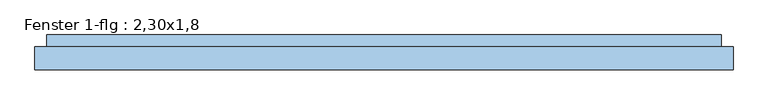
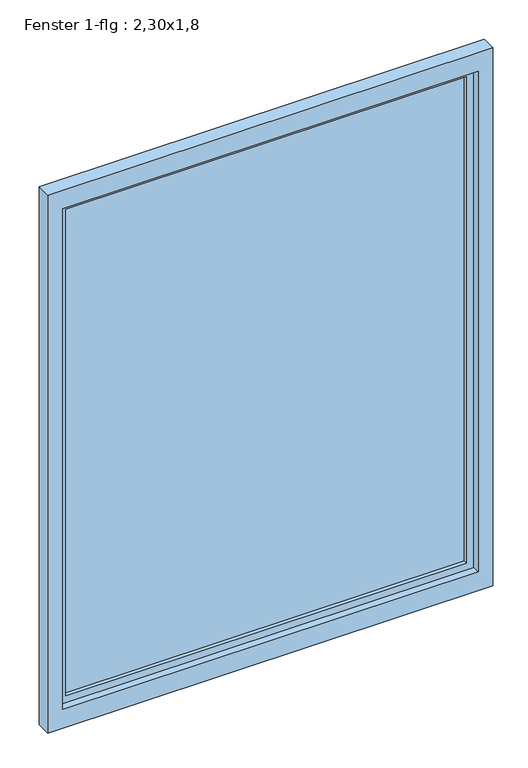
"""IFC4 building model written with IfcOpenShell, lengths in millimetres: window geometry, Fenster 1-flg : 2,30x1,8."""

import ifcopenshell
import ifcopenshell.guid

model = None  # the IFC model being written
_history = None  # IfcOwnerHistory: only IFC2X3 demands one
_inside = {}  # id of a spatial element -> (the spatial element, [elements in it])
_under = {}  # id of a project, library or spatial element -> (it, [spatial elements below it])
_declared = {}  # id of a project -> (the project, [libraries it declares])
_typed = {}  # id of a type object -> (the type object, [elements of that type])
_made_of = {}  # id of a material, layer set ... -> (it, [elements and type objects made of it])


def new_model(schema):
    """Start an empty IFC model of exactly this schema.

    Asked for "IFC4X3", IfcOpenShell would pick the latest addendum, in which some entities
    have other attributes; the version numbers below select the first issue.
    IFC2X3 requires an IfcOwnerHistory on every rooted entity: one is made here for all.
    """
    global model, _history
    if schema == "IFC4X3":
        model = ifcopenshell.file(schema_version=(4, 3, 0, 0))
    else:
        model = ifcopenshell.file(schema=schema)
    _inside.clear()
    _under.clear()
    _declared.clear()
    _typed.clear()
    _made_of.clear()
    _history = None
    if model.schema == "IFC2X3":
        org = make("IfcOrganization", Name="unknown")
        user = make(
            "IfcPersonAndOrganization",
            ThePerson=make("IfcPerson", FamilyName="unknown"),
            TheOrganization=org,
        )
        app = make(
            "IfcApplication",
            ApplicationDeveloper=org,
            Version="unknown",
            ApplicationFullName="unknown",
            ApplicationIdentifier="unknown",
        )
        _history = make(
            "IfcOwnerHistory",
            OwningUser=user,
            OwningApplication=app,
            ChangeAction="ADDED",
            CreationDate=0,
        )
    return model


def make(cls, **values):
    """One entity of the class cls with the attributes given. An attribute that is None is left unset."""
    return model.create_entity(
        cls, **{name: value for name, value in values.items() if value is not None}
    )


def rooted(cls, **values):
    """An entity with a GlobalId (a new one), such as an element, a storey or a relation."""
    return make(cls, GlobalId=ifcopenshell.guid.new(), OwnerHistory=_history, **values)


def si_unit(unit_type, name, prefix=None):
    """IfcSIUnit, for example si_unit("LENGTHUNIT", "METRE", prefix="MILLI")."""
    return make("IfcSIUnit", UnitType=unit_type, Prefix=prefix, Name=name)


def assignment(units):
    """IfcUnitAssignment: the units of a project."""
    return None if units is None else make("IfcUnitAssignment", Units=units)


def point(xyz):
    """IfcCartesianPoint."""
    return None if xyz is None else make("IfcCartesianPoint", Coordinates=xyz)


def direction(xyz):
    """IfcDirection."""
    return None if xyz is None else make("IfcDirection", DirectionRatios=xyz)


def frame(location, z_axis=None, x_axis=None):
    """IfcAxis2Placement3D, a coordinate frame: its origin and axes. An axis left out is left unset."""
    return make(
        "IfcAxis2Placement3D",
        Location=point(location),
        Axis=direction(z_axis),
        RefDirection=direction(x_axis),
    )


def origin():
    """The frame at (0, 0, 0) with its axes left unset."""
    return frame((0.0, 0.0, 0.0))


def place(relative_to, where):
    """IfcLocalPlacement: puts the frame where relative to a parent placement (None: the world)."""
    return make(
        "IfcLocalPlacement", PlacementRelTo=relative_to, RelativePlacement=where
    )


def context(
    kind, dimensions, precision=None, world=None, true_north=None, identifier=None
):
    """IfcGeometricRepresentationContext, for example the 3D "Model" context."""
    return make(
        "IfcGeometricRepresentationContext",
        ContextIdentifier=identifier,
        ContextType=kind,
        CoordinateSpaceDimension=dimensions,
        Precision=precision,
        WorldCoordinateSystem=world,
        TrueNorth=true_north,
    )


def project(units=None, contexts=None):
    """IfcProject with its units and contexts."""
    return rooted(
        "IfcProject",
        Name="project",
        RepresentationContexts=contexts,
        UnitsInContext=assignment(units),
    )


def spatial(cls, under=None, at=None, **own):
    """A site, building, storey or space (cls), placed at a placement, below another one or the project."""
    s = rooted(cls, ObjectPlacement=at, **own)
    if under is not None:
        _under.setdefault(under.id(), (under, []))[1].append(s)
    return s


def polyline(points):
    """IfcPolyline through the points."""
    return make("IfcPolyline", Points=[point(p) for p in points])


def outline(outer, holes=None, kind="AREA"):
    """IfcArbitraryClosedProfileDef: a profile drawn as a closed curve; with holes, ...WithVoids."""
    if holes is None:
        return make("IfcArbitraryClosedProfileDef", ProfileType=kind, OuterCurve=outer)
    return make(
        "IfcArbitraryProfileDefWithVoids",
        ProfileType=kind,
        OuterCurve=outer,
        InnerCurves=holes,
    )


def extrude(swept, where, along, depth):
    """IfcExtrudedAreaSolid: the profile swept, set in the frame where, extruded along a direction by depth."""
    return make(
        "IfcExtrudedAreaSolid",
        SweptArea=swept,
        Position=where,
        ExtrudedDirection=direction(along),
        Depth=depth,
    )


def faces_of(points, faces, orient=None, outer=None):
    """IfcFace entities. A face is a list of loops; a loop is a list of indices into points, from 0.

    orient and outer hold one flag for each loop. By default every Orientation is true, the
    first loop of a face is its IfcFaceOuterBound and the others are IfcFaceBound.
    """
    made = []
    for i, loops in enumerate(faces):
        bounds = []
        for j, loop in enumerate(loops):
            is_outer = j == 0 if outer is None else outer[i][j]
            bounds.append(
                make(
                    "IfcFaceOuterBound" if is_outer else "IfcFaceBound",
                    Bound=make("IfcPolyLoop", Polygon=[points[k] for k in loop]),
                    Orientation=True if orient is None else orient[i][j],
                )
            )
        made.append(make("IfcFace", Bounds=bounds))
    return made


def faceted_brep(points, faces, orient=None, outer=None, voids=None):
    """IfcFacetedBrep: a solid bounded by flat faces; with voids (closed shells), ...WithVoids."""
    shared = [point(p) for p in points]
    hull = make("IfcClosedShell", CfsFaces=faces_of(shared, faces, orient, outer))
    if voids is None:
        return make("IfcFacetedBrep", Outer=hull)
    return make(
        "IfcFacetedBrepWithVoids",
        Outer=hull,
        Voids=[
            make(cls, CfsFaces=faces_of(shared, fs, o, b)) for cls, fs, o, b in voids
        ],
    )


def shape(context_of_items, identifier, shape_type, items):
    """IfcShapeRepresentation: the items that make up one representation, for example the "Body"."""
    return make(
        "IfcShapeRepresentation",
        ContextOfItems=context_of_items,
        RepresentationIdentifier=identifier,
        RepresentationType=shape_type,
        Items=items,
    )


def source(mapping_origin, context_of_items, identifier, shape_type, items):
    """IfcRepresentationMap: a shape defined once, which mapped items show again and again."""
    return make(
        "IfcRepresentationMap",
        MappingOrigin=mapping_origin,
        MappedRepresentation=shape(context_of_items, identifier, shape_type, items),
    )


def transform(
    local_origin,
    x_axis=None,
    y_axis=None,
    z_axis=None,
    scale=None,
    scale2=None,
    scale3=None,
    uniform=True,
):
    """IfcCartesianTransformationOperator3D, or its non-uniform kind. x_axis, y_axis, z_axis: its Axis1, 2, 3."""
    if uniform:
        return make(
            "IfcCartesianTransformationOperator3D",
            Axis1=direction(x_axis),
            Axis2=direction(y_axis),
            LocalOrigin=point(local_origin),
            Scale=scale,
            Axis3=direction(z_axis),
        )
    return make(
        "IfcCartesianTransformationOperator3DnonUniform",
        Axis1=direction(x_axis),
        Axis2=direction(y_axis),
        LocalOrigin=point(local_origin),
        Scale=scale,
        Axis3=direction(z_axis),
        Scale2=scale2,
        Scale3=scale3,
    )


def mapped(mapping_source, mapping_target):
    """IfcMappedItem: shows the shape of a source again, moved by a transform."""
    return make(
        "IfcMappedItem", MappingSource=mapping_source, MappingTarget=mapping_target
    )


def made_of(thing, what):
    """Note that an element or type object is made of a material, layer set ...; save() writes the relation."""
    if what is not None:
        _made_of.setdefault(what.id(), (what, []))[1].append(thing)
    return thing


def element(
    cls,
    number,
    at=None,
    inside=None,
    cuts=None,
    type_object=None,
    material=None,
    context=None,
    identifier="Body",
    shape_type=None,
    held_by="IfcProductDefinitionShape",
    body=None,
    shapes=None,
    **own,
):
    """One element of the class cls, such as IfcWall. Its Tag is "e" and its number.

    at: its placement. inside: the storey or other place that contains it. cuts: it is an
    opening in that element (IfcRelVoidsElement). A single representation is given by context,
    identifier, shape_type and body (its items); several are given by shapes. held_by: the class
    of the entity that holds the representations. save() writes the other relations.
    """
    e = rooted(cls, Tag="e%d" % number, ObjectPlacement=at, **own)
    if body is not None:
        shapes = [shape(context, identifier, shape_type, body)]
    if shapes is not None:
        e.Representation = make(held_by, Representations=shapes)
    if inside is not None:
        _inside.setdefault(inside.id(), (inside, []))[1].append(e)
    if cuts is not None:
        rooted(
            "IfcRelVoidsElement", RelatingBuildingElement=cuts, RelatedOpeningElement=e
        )
    if type_object is not None:
        _typed.setdefault(type_object.id(), (type_object, []))[1].append(e)
    return made_of(e, material)


def aggregate(whole, parts):
    """IfcRelAggregates: a whole, such as a stair, and the parts it consists of."""
    return rooted("IfcRelAggregates", RelatingObject=whole, RelatedObjects=parts)


def save(model, path):
    """Write the relations noted so far, then the file.

    IfcRelAggregates (storeys below a building ...), IfcRelContainedInSpatialStructure (elements
    in a storey), IfcRelDefinesByType, IfcRelAssociatesMaterial and IfcRelDeclares: one each for
    every whole, place, type object, material and project.
    """
    for whole, parts in _under.values():
        aggregate(whole, parts)
    for where, things in _inside.values():
        rooted(
            "IfcRelContainedInSpatialStructure",
            RelatedElements=things,
            RelatingStructure=where,
        )
    for kind, things in _typed.values():
        rooted("IfcRelDefinesByType", RelatedObjects=things, RelatingType=kind)
    for what, things in _made_of.values():
        rooted("IfcRelAssociatesMaterial", RelatedObjects=things, RelatingMaterial=what)
    for by, libraries in _declared.values():
        rooted("IfcRelDeclares", RelatingContext=by, RelatedDefinitions=libraries)
    model.write(path)


def fenster_1_flg_2_30x1_8_4fa574a4(model_context):
    return source(origin(), model_context, "Body", "SolidModel", [
        extrude(outline(polyline([(3300.0, 900.0), (3300.0, -900.0), (1000.0, -900.0), (1000.0, 900.0), (3300.0, 900.0)]), holes=[polyline([(3220.0, 840.0), (1080.0, 840.0), (1080.0, -840.0), (3220.0, -840.0), (3220.0, 840.0)])]), frame((0.0, -30.0, 0.0), z_axis=(0.0, 1.0, 0.0), x_axis=(0.0, 0.0, 1.0)), (0.0, 0.0, 1.0), 60.0),
        faceted_brep([(870.0, 30.0, 3250.0), (870.0, 30.0, 1050.0), (870.0, 60.0, 1050.0), (870.0, 60.0, 3250.0), (-870.0, 60.0, 1050.0), (-870.0, 60.0, 3250.0), (810.0, 60.0, 1110.0), (810.0, 60.0, 3190.0), (-810.0, 60.0, 3190.0), (-810.0, 60.0, 1110.0), (-870.0, 30.0, 1050.0), (-870.0, 30.0, 3250.0), (840.0, 30.0, 3220.0), (840.0, 30.0, 1080.0), (-840.0, 30.0, 1080.0), (-840.0, 30.0, 3220.0), (840.0, 0.0, 3220.0), (840.0, 0.0, 1080.0), (-840.0, 0.0, 1080.0), (-840.0, 0.0, 3220.0), (810.0, 0.0, 3190.0), (810.0, 0.0, 1110.0), (-810.0, 0.0, 1110.0), (-810.0, 0.0, 3190.0)], [[[0, 1, 2, 3]], [[3, 2, 4, 5], [6, 7, 8, 9]], [[1, 10, 4, 2]], [[1, 0, 11, 10], [12, 13, 14, 15]], [[16, 17, 13, 12]], [[17, 18, 14, 13]], [[17, 16, 19, 18], [20, 21, 22, 23]], [[7, 6, 21, 20]], [[6, 9, 22, 21]], [[10, 11, 5, 4]], [[18, 19, 15, 14]], [[9, 8, 23, 22]], [[11, 0, 3, 5]], [[19, 16, 12, 15]], [[8, 7, 20, 23]]]),
        extrude(outline(polyline([(810.0, 45.0), (810.0, 15.0), (-810.0, 15.0), (-810.0, 45.0), (810.0, 45.0)])), frame((0.0, 0.0, 1110.0), z_axis=(0.0, 0.0, 1.0), x_axis=(1.0, 0.0, 0.0)), (0.0, 0.0, 1.0), 2080.0),
    ])


if __name__ == "__main__":
    model = new_model("IFC4")
    model_context = context("Model", 3, world=origin())
    ifc_project = project(units=[si_unit("LENGTHUNIT", "METRE", prefix="MILLI")], contexts=[model_context])
    site = spatial("IfcSite", under=ifc_project)
    building = spatial("IfcBuilding", under=site)
    placement = place(None, origin())
    fenster_1_flg_2_30x1_8_shape = fenster_1_flg_2_30x1_8_4fa574a4(model_context)
    element("IfcWindow", 1, ObjectType="Fenster 1-flg : 2,30x1,8", at=placement, inside=building, context=model_context, shape_type="MappedRepresentation", body=[
        mapped(fenster_1_flg_2_30x1_8_shape, transform((0.0, 0.0, 0.0), x_axis=(1.0, 0.0, 0.0), y_axis=(0.0, 1.0, 0.0), z_axis=(0.0, 0.0, 1.0))),
    ])
    save(model, "model.ifc")

# Revit data of these elements
# Type "Fenster 1-flg : 2,30x1,8"
#   Type Mark = "71"
#   Operation = "SinglePanel"
#   Keynote = "16.05.01"
#   Visual Light Transmittance = 0.9
#   Solar Heat Gain Coefficient = 0.86
#   Rough Width = 1.800 m
#   Rough Height = 2.300 m
#   Heat Transfer Coefficient (U) = 5.5617 W/(m²·K)
#   Rahmentiefe = 0.060 m
#   Rahmenhöhe - unten = 0.080 m
#   Rahmenhöhe - oben = 0.080 m
#   Rahmenbreite = 0.060 m
#   Height = 2.300 m
#   Tiefe Flügel = 0.060 m
#   Flügelbreite = 0.060 m
#   Einbautiefe (von außen) [instance default] = 0.100 m
#   Width = 1.800 m
#   Klappflügel [instance default] = no
#   Kippflügel [instance default] = yes
#   Öffnungsrichtung in Draufsicht anzeigen [instance default] = no
#   Drehflügel 1 [instance default] = yes
#   Rahmen 1 [instance default] = none
#   Glas [instance default] = none
#   Flügel [instance default] = none
#   Fensterbank Innenseite [instance default] = none
#   Fensterbank Außenseite [instance default] = none
#   Construction Type Id = ""
#   Wall Closure = (empty or 0)
#   Analytic Construction = (empty or 0)
# Element 1 (IfcWindow, "Fenster 1-flg : 2,30x1,8")
#   Einbautiefe (von außen) = 0.120 m
#   Materials on its faces: "Kunststoff - Weiß", "Glas"
# Materials
#   "Kunststoff - Weiß": class "Kunststoff", colour RGB 249 249 249, transparency 0, Cost = 0
#   "Glas": class "Glas", colour RGB 0 0 255, transparency 0.75, Comments = "Render-Darstellung nicht aktualisiert ", Cost = 0
